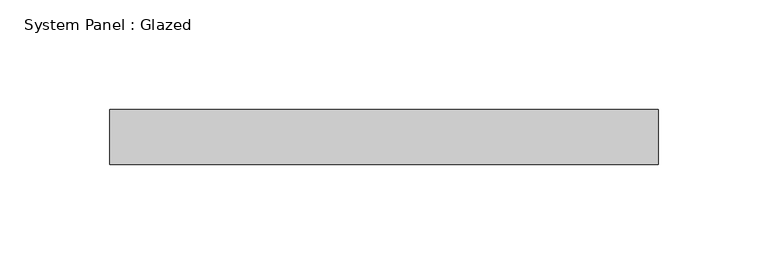
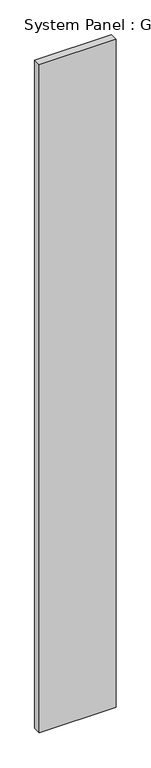
"""IFC4 building model written with IfcOpenShell, lengths in millimetres: plate geometry, System Panel : Glazed."""

from ifc_helpers import new_model, si_unit, origin, origin_with_axes, place, context, project, spatial, polyline, outline, extrude, source, transform, mapped, element, save


def system_panel_glazed_27ab1db5(model_context):
    return source(origin(), model_context, "Body", "SweptSolid", [
        extrude(outline(polyline([(125.0000001, 24.5), (-125.0000001, 24.5), (-125.0000001, 49.5), (125.0000001, 49.5), (125.0000001, 24.5)])), origin_with_axes(), (0.0, 0.0, 1.0), 2300.0),
    ])


if __name__ == "__main__":
    model = new_model("IFC4")
    model_context = context("Model", 3, world=origin())
    ifc_project = project(units=[si_unit("LENGTHUNIT", "METRE", prefix="MILLI")], contexts=[model_context])
    site = spatial("IfcSite", under=ifc_project)
    building = spatial("IfcBuilding", under=site)
    placement = place(None, origin())
    system_panel_glazed_shape = system_panel_glazed_27ab1db5(model_context)
    element("IfcPlate", 1, ObjectType="System Panel : Glazed", at=placement, inside=building, context=model_context, shape_type="MappedRepresentation", body=[
        mapped(system_panel_glazed_shape, transform((0.0, 0.0, 0.0), x_axis=(1.0, 0.0, 0.0), y_axis=(0.0, 1.0, 0.0), z_axis=(0.0, 0.0, 1.0))),
    ])
    save(model, "model.ifc")

# Revit data of these elements
# Type "System Panel : Glazed"
#   Construction Type Id = "GSP4R"
#   Analytic Construction = "1/8 in Pilkington single glazing"
#   Visual Light Transmittance = 0.9
#   Solar Heat Gain Coefficient = 0.86
#   Heat Transfer Coefficient (U) = 6.7069 W/(m²·K)
#   Define Thermal Properties by = 1
# Element 1 (IfcPlate, "System Panel : Glazed")
#   Materials on its faces: "Glass"
# Materials
#   "Glass": class "Glass", colour RGB 0 128 192, transparency 0.9, Description = "Soda Lime Glass", Cost = 0
